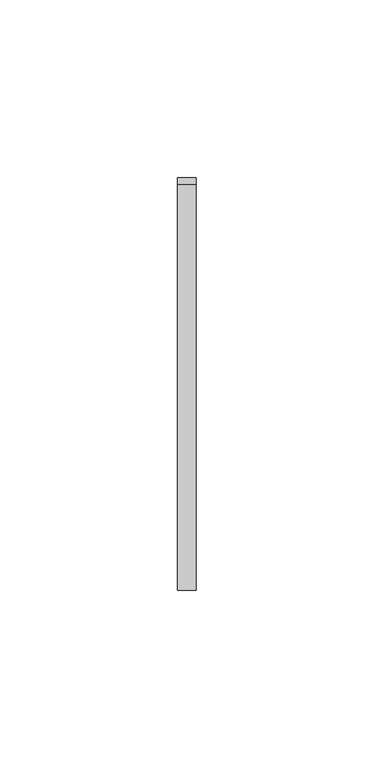
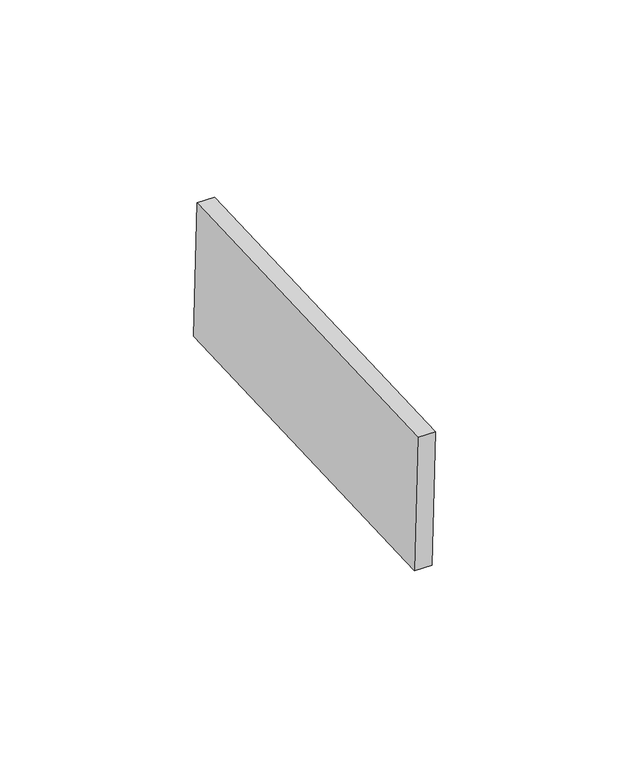
"""IFC4 building model written with IfcOpenShell, lengths in millimetres: proxy geometry, Inner panel:Inner panel:1:Inner panel:1 : Inner panel:Inner panel:300324:2:Inner panel:1:Inner panel:1 : Inner panel:Inner panel:300324:2 : Inner panel:Inner panel:1:Inner panel:1 : Inner panel:Inner panel:300324:300043:28 : Inner panel:Inner panel:1:Inner panel:1 : Inner panel:Inner panel:300324:2:Inner panel:1:Inner panel:1 : Inner panel:Inner panel:300324:2 : Inner panel:Inner panel:1:Inner panel:1 : Inner panel:Inner panel:300324:300043:308120."""

from ifc_helpers import new_model, si_unit, frame, origin, place, context, project, spatial, polyline, outline, extrude, source, transform, mapped, element, save


def generic_models_5cf26771(model_context):
    return source(origin(), model_context, "Body", "SweptSolid", [
        extrude(outline(polyline([(0.0, -114.3), (0.0, 0.0), (5.2138089, 0.0), (5.2138089, -114.3), (0.0, -114.3)])), frame((593530.195117, -578297.797364, 3981.6641254), z_axis=(0.0, -0.04163054471216399, 0.9991330730923527), x_axis=(-1.0, 0.0, 0.0)), (0.0, 0.0, 1.0), 43.2233908),
    ])


if __name__ == "__main__":
    model = new_model("IFC4")
    model_context = context("Model", 3, world=origin())
    ifc_project = project(units=[si_unit("LENGTHUNIT", "METRE", prefix="MILLI")], contexts=[model_context])
    site = spatial("IfcSite", under=ifc_project)
    building = spatial("IfcBuilding", under=site)
    placement = place(None, origin())
    generic_models_shape = generic_models_5cf26771(model_context)
    element("IfcBuildingElementProxy", 1, Name="Inner panel:Inner panel:1:Inner panel:1 : Inner panel:Inner panel:300324:2:Inner panel:1:Inner panel:1 : Inner panel:Inner panel:300324:2 : Inner panel:Inner panel:1:Inner panel:1 : Inner panel:Inner panel:300324:300043:28 : Inner panel:Inner panel:1:Inner panel:1 : Inner panel:Inner panel:300324:2:Inner panel:1:Inner panel:1 : Inner panel:Inner panel:300324:2 : Inner panel:Inner panel:1:Inner panel:1 : Inner panel:Inner panel:300324:300043:308120", ObjectType="Inner panel:Inner panel:1:Inner panel:1 : Inner panel:Inner panel:300324:2:Inner panel:1:Inner panel:1 : Inner panel:Inner panel:300324:2 : Inner panel:Inner panel:1:Inner panel:1 : Inner panel:Inner panel:300324:300043:28 : Inner panel:Inner panel:1:Inner panel:1 : Inner panel:Inner panel:300324:2:Inner panel:1:Inner panel:1 : Inner panel:Inner panel:300324:2 : Inner panel:Inner panel:1:Inner panel:1 : Inner panel:Inner panel:300324:300043:308120", at=placement, inside=building, context=model_context, shape_type="MappedRepresentation", body=[
        mapped(generic_models_shape, transform((0.0, 0.0, 0.0), x_axis=(1.0, 0.0, 0.0), y_axis=(0.0, 1.0, 0.0), z_axis=(0.0, 0.0, 1.0))),
    ])
    save(model, "model.ifc")

# Revit data of these elements
# Type "Inner panel:Inner panel:1:Inner panel:1 : Inner panel:Inner panel:300324:2:Inner panel:1:Inner panel:1 : Inner panel:Inner panel:300324:2 : Inner panel:Inner panel:1:Inner panel:1 : Inner panel:Inner panel:300324:300043:28 : Inner panel:Inner panel:1:Inner panel:1 : Inner panel:Inner panel:300324:2:Inner panel:1:Inner panel:1 : Inner panel:Inner panel:300324:2 : Inner panel:Inner panel:1:Inner panel:1 : Inner panel:Inner panel:300324:300043:308120"
#   NameOverride = "Inner panel:Inner panel:1:Inner panel:1 : Inner panel:Inner panel:300324:2:Inner panel:1:Inner panel:1 : Inner panel:Inner panel:300324:2 : Inner panel:Inner panel:1:Inner panel:1 : Inner panel:Inner panel:300324:300043:308120"
#   ObjectTypeOverride = "Inner panel:1:Inner panel:1 : Inner panel:Inner panel:300324:2 : Inner panel:Inner panel:1:Inner panel:1 : Inner panel:Inner panel:300324:300043"
#   Reference = "Inner panel"
#   Tag = "308120"
# Element 1 (IfcBuildingElementProxy, "Inner panel:Inner panel:1:Inner panel:1 : Inner panel:Inner panel:300324:2:Inner panel:1:Inner panel:1 : Inner panel:Inner panel:300324:2 : Inner panel:Inner panel:1:Inner panel:1 : Inner panel:Inner panel:300324:300043:28 : Inner panel:Inner panel:1:Inner panel:1 : Inner panel:Inner panel:300324:2:Inner panel:1:Inner panel:1 : Inner panel:Inner panel:300324:2 : Inner panel:Inner panel:1:Inner panel:1 : Inner panel:Inner panel:300324:300043:308120")
#   Materials on its faces: "SLIDING CLIP"
# Materials
#   "SLIDING CLIP": class "Generic", colour RGB 120 120 120, transparency 0, Cost = 0
